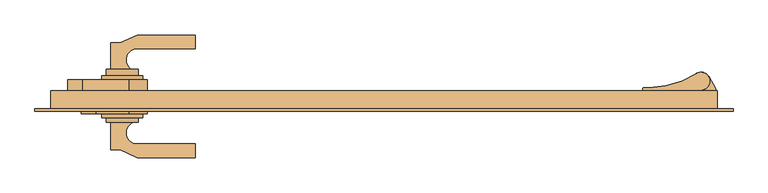
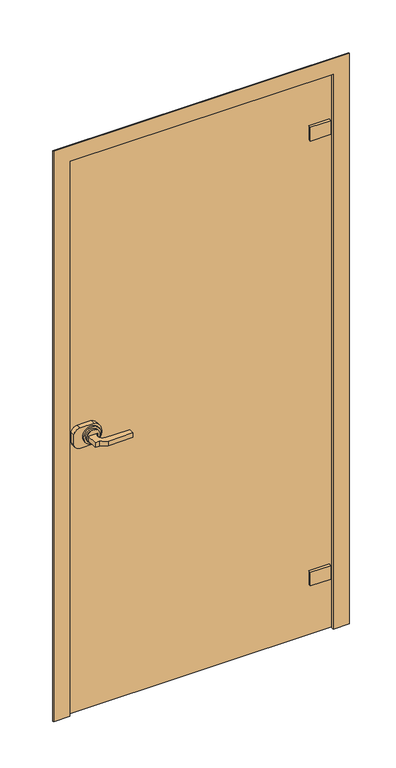
"""IFC4 building model written with IfcOpenShell, lengths in millimetres: door geometry, Doors_Doors_Faraone_Anta : Doors_Doors_Faraone_Anta."""

from ifc_helpers import new_model, si_unit, point, frame, frame_2d, origin, place, context, project, spatial, polyline, circle_curve, trimmed, segment, composite_curve, outline, extrude, faceted_brep, source, transform, mapped, element, save


def door_6f7413cf(model_context):
    return source(origin(), model_context, "Body", "SolidModel", [
        extrude(outline(polyline([(376.5509112, -11.599726), (376.5509112, -1.8997991), (446.250386, -1.8997991), (446.250386, -11.599726), (376.5509112, -11.599726)])), frame((0.0, 0.0, 1799.0000277), z_axis=(0.0, 0.0, 1.0), x_axis=(1.0, 0.0, 0.0)), (0.0, 0.0, 1.0), 50.0),
        extrude(outline(composite_curve([segment(trimmed(circle_curve(frame_2d((378.5508961, 17.600054)), 1.9999849), [point((376.5509112, 17.600054))], [point((378.5508961, 19.6000389))], False, "CARTESIAN"), True, "CONTINUOUS"), segment(polyline([(378.5508961, 19.6000389), (386.5508359, 19.6000389)]), True, "CONTINUOUS"), segment(trimmed(circle_curve(frame_2d((385.1363002, 147.5843675)), 127.9921454), [point((386.5508359, 19.6000389))], [point((454.7624862, 40.1870515))], True, "CARTESIAN"), True, "CONTINUOUS"), segment(trimmed(circle_curve(frame_2d((461.5502708, 29.0999673)), 12.9999021), [point((454.7624862, 40.1870515))], [point((466.1896331, 16.9560894))], False, "CARTESIAN"), True, "CONTINUOUS"), segment(polyline([(466.1896331, 16.9560894), (446.5503838, 9.6001143), (446.5503838, 8.1001256), (376.5509112, 8.1001256), (376.5509112, 17.600054)]), True, "CONTINUOUS")], self_intersect=False)), frame((0.0, 0.0, 1799.0000277), z_axis=(0.0, 0.0, 1.0), x_axis=(1.0, 0.0, 0.0)), (0.0, 0.0, 1.0), 50.0),
        extrude(outline(composite_curve([segment(polyline([(483.3501065, 18.0609582), (483.3501065, 15.0000736), (461.5537493, 15.0000736), (457.1671339, 16.861276)]), True, "CONTINUOUS"), segment(trimmed(circle_curve(frame_2d((461.5502708, 29.0999673)), 12.9999021), [point((457.1671339, 16.861276))], [point((451.2009633, 36.9669419))], False, "CARTESIAN"), True, "CONTINUOUS"), segment(trimmed(circle_curve(frame_2d((461.5502708, 29.0999673)), 12.9999021), [point((451.2009633, 36.9669419))], [point((472.573012, 35.9917471))], False, "CARTESIAN"), True, "CONTINUOUS"), segment(polyline([(472.573012, 35.9917471), (483.3501065, 18.0609582)]), True, "CONTINUOUS")], self_intersect=False)), frame((0.0, 0.0, 1749.0000277), z_axis=(0.0, 0.0, 1.0), x_axis=(1.0, 0.0, 0.0)), (0.0, 0.0, 1.0), 50.0),
        extrude(outline(polyline([(376.5509112, -11.599726), (376.5509112, -1.8997991), (446.250386, -1.8997991), (446.250386, -11.599726), (376.5509112, -11.599726)])), frame((0.0, 0.0, 182.0), z_axis=(0.0, 0.0, 1.0), x_axis=(1.0, 0.0, 0.0)), (0.0, 0.0, 1.0), 50.0),
        extrude(outline(composite_curve([segment(trimmed(circle_curve(frame_2d((378.5508961, 17.600054)), 1.9999849), [point((376.5509112, 17.600054))], [point((378.5508961, 19.6000389))], False, "CARTESIAN"), True, "CONTINUOUS"), segment(polyline([(378.5508961, 19.6000389), (386.5508359, 19.6000389)]), True, "CONTINUOUS"), segment(trimmed(circle_curve(frame_2d((385.1363002, 147.5843675)), 127.9921454), [point((386.5508359, 19.6000389))], [point((454.7624862, 40.1870515))], True, "CARTESIAN"), True, "CONTINUOUS"), segment(trimmed(circle_curve(frame_2d((461.5502708, 29.0999673)), 12.9999021), [point((454.7624862, 40.1870515))], [point((466.1896331, 16.9560894))], False, "CARTESIAN"), True, "CONTINUOUS"), segment(polyline([(466.1896331, 16.9560894), (446.5503838, 9.6001143), (446.5503838, 8.1001256), (376.5509112, 8.1001256), (376.5509112, 17.600054)]), True, "CONTINUOUS")], self_intersect=False)), frame((0.0, 0.0, 182.0), z_axis=(0.0, 0.0, 1.0), x_axis=(1.0, 0.0, 0.0)), (0.0, 0.0, 1.0), 50.0),
        extrude(outline(composite_curve([segment(polyline([(483.3501065, 18.0609582), (483.3501065, 15.0000736), (461.5537493, 15.0000736), (457.1671339, 16.861276)]), True, "CONTINUOUS"), segment(trimmed(circle_curve(frame_2d((461.5502708, 29.0999673)), 12.9999021), [point((457.1671339, 16.861276))], [point((451.2009633, 36.9669419))], False, "CARTESIAN"), True, "CONTINUOUS"), segment(trimmed(circle_curve(frame_2d((461.5502708, 29.0999673)), 12.9999021), [point((451.2009633, 36.9669419))], [point((472.573012, 35.9917471))], False, "CARTESIAN"), True, "CONTINUOUS"), segment(polyline([(472.573012, 35.9917471), (483.3501065, 18.0609582)]), True, "CONTINUOUS")], self_intersect=False)), frame((0.0, 0.0, 132.0), z_axis=(0.0, 0.0, 1.0), x_axis=(1.0, 0.0, 0.0)), (0.0, 0.0, 1.0), 50.0),
        extrude(outline(composite_curve([segment(trimmed(circle_curve(frame_2d((1003.2884985, -381.2459675)), 23.0897305), [point((1003.2884985, -404.335698))], [point((1003.2884985, -358.156237))], False, "CARTESIAN"), True, "CONTINUOUS"), segment(trimmed(circle_curve(frame_2d((1003.2884985, -381.2459675)), 23.0897305), [point((1003.2884985, -358.156237))], [point((1003.2884985, -404.335698))], False, "CARTESIAN"), True, "CONTINUOUS")], self_intersect=False)), frame((0.0, 36.9863146, 0.0), z_axis=(0.0, 1.0, 0.0), x_axis=(0.0, 0.0, 1.0)), (0.0, 0.0, 1.0), 9.3686894),
        extrude(outline(composite_curve([segment(trimmed(circle_curve(frame_2d((987.7717852, -438.83347)), 22.4105262), [point((983.5880679, -460.8500137))], [point((965.361259, -438.83347))], False, "CARTESIAN"), True, "CONTINUOUS"), segment(polyline([(965.361259, -438.83347), (965.361259, -373.83347)]), True, "CONTINUOUS"), segment(trimmed(circle_curve(frame_2d((1002.861259, -383.4990023)), 38.7256054), [point((965.361259, -373.83347))], [point((1039.5100566, -370.9874819))], False, "CARTESIAN"), True, "CONTINUOUS"), segment(polyline([(1039.5100566, -370.9874819), (1039.5100566, -438.83347)]), True, "CONTINUOUS"), segment(trimmed(circle_curve(frame_2d((1017.0995304, -438.83347)), 22.4105262), [point((1039.5100566, -438.83347))], [point((1021.2832478, -460.8500137))], False, "CARTESIAN"), True, "CONTINUOUS"), segment(polyline([(1021.2832478, -460.8500137), (983.5880679, -460.8500137)]), True, "CONTINUOUS")], self_intersect=False)), frame((0.0, 8.1001256, 0.0), z_axis=(0.0, 1.0, 0.0), x_axis=(0.0, 0.0, 1.0)), (0.0, 0.0, 1.0), 23.0652027),
        extrude(outline(composite_curve([segment(trimmed(circle_curve(frame_2d((987.7717852, -438.83347)), 22.4105262), [point((983.5880679, -460.8500137))], [point((965.361259, -438.83347))], False, "CARTESIAN"), True, "CONTINUOUS"), segment(polyline([(965.361259, -438.83347), (965.361259, -373.83347)]), True, "CONTINUOUS"), segment(trimmed(circle_curve(frame_2d((1002.861259, -383.4990023)), 38.7256054), [point((965.361259, -373.83347))], [point((1039.5100566, -370.9874819))], False, "CARTESIAN"), True, "CONTINUOUS"), segment(polyline([(1039.5100566, -370.9874819), (1039.5100566, -438.83347)]), True, "CONTINUOUS"), segment(trimmed(circle_curve(frame_2d((1017.0995304, -438.83347)), 22.4105262), [point((1039.5100566, -438.83347))], [point((1021.2832478, -460.8500137))], False, "CARTESIAN"), True, "CONTINUOUS"), segment(polyline([(1021.2832478, -460.8500137), (983.5880679, -460.8500137)]), True, "CONTINUOUS")], self_intersect=False)), frame((0.0, 8.1001256, 0.0), z_axis=(0.0, 1.0, 0.0), x_axis=(0.0, 0.0, 1.0)), (0.0, 0.0, 1.0), 23.0652027),
        extrude(outline(composite_curve([segment(trimmed(circle_curve(frame_2d((1003.2884985, -381.2459675)), 30.0), [point((1003.2884985, -411.2459675))], [point((1003.2884985, -351.2459675))], False, "CARTESIAN"), True, "CONTINUOUS"), segment(trimmed(circle_curve(frame_2d((1003.2884985, -381.2459675)), 30.0), [point((1003.2884985, -351.2459675))], [point((1003.2884985, -411.2459675))], False, "CARTESIAN"), True, "CONTINUOUS")], self_intersect=False)), frame((0.0, 31.1653283, 0.0), z_axis=(0.0, 1.0, 0.0), x_axis=(0.0, 0.0, 1.0)), (0.0, 0.0, 1.0), 5.8209863),
        extrude(outline(composite_curve([segment(trimmed(circle_curve(frame_2d((987.7717852, -438.83347)), 22.4105262), [point((983.5880679, -460.8500137))], [point((965.361259, -438.83347))], False, "CARTESIAN"), True, "CONTINUOUS"), segment(polyline([(965.361259, -438.83347), (965.361259, -373.83347)]), True, "CONTINUOUS"), segment(trimmed(circle_curve(frame_2d((1002.861259, -383.4990023)), 38.7256054), [point((965.361259, -373.83347))], [point((1039.5100566, -370.9874819))], False, "CARTESIAN"), True, "CONTINUOUS"), segment(polyline([(1039.5100566, -370.9874819), (1039.5100566, -438.83347)]), True, "CONTINUOUS"), segment(trimmed(circle_curve(frame_2d((1017.0995304, -438.83347)), 22.4105262), [point((1039.5100566, -438.83347))], [point((1021.2832478, -460.8500137))], False, "CARTESIAN"), True, "CONTINUOUS"), segment(polyline([(1021.2832478, -460.8500137), (983.5880679, -460.8500137)]), True, "CONTINUOUS")], self_intersect=False)), frame((0.0, 8.1001256, 0.0), z_axis=(0.0, 1.0, 0.0), x_axis=(0.0, 0.0, 1.0)), (0.0, 0.0, 1.0), 23.0652027),
        extrude(outline(composite_curve([segment(trimmed(circle_curve(frame_2d((1003.2884985, -381.2459675)), 23.0897305), [point((1003.2884985, -404.335698))], [point((1003.2884985, -358.156237))], False, "CARTESIAN"), True, "CONTINUOUS"), segment(trimmed(circle_curve(frame_2d((1003.2884985, -381.2459675)), 23.0897305), [point((1003.2884985, -358.156237))], [point((1003.2884985, -404.335698))], False, "CARTESIAN"), True, "CONTINUOUS")], self_intersect=False)), frame((0.0, 32.1653283, 0.0), z_axis=(0.0, 1.0, 0.0), x_axis=(0.0, 0.0, 1.0)), (0.0, 0.0, 1.0), 14.1896757),
        extrude(outline(composite_curve([segment(trimmed(circle_curve(frame_2d((987.7717852, -438.83347)), 22.4105262), [point((983.5880679, -460.8500137))], [point((965.361259, -438.83347))], False, "CARTESIAN"), True, "CONTINUOUS"), segment(polyline([(965.361259, -438.83347), (965.361259, -373.83347)]), True, "CONTINUOUS"), segment(trimmed(circle_curve(frame_2d((1002.861259, -383.4990023)), 38.7256054), [point((965.361259, -373.83347))], [point((1039.5100566, -370.9874819))], False, "CARTESIAN"), True, "CONTINUOUS"), segment(polyline([(1039.5100566, -370.9874819), (1039.5100566, -438.83347)]), True, "CONTINUOUS"), segment(trimmed(circle_curve(frame_2d((1017.0995304, -438.83347)), 22.4105262), [point((1039.5100566, -438.83347))], [point((1021.2832478, -460.8500137))], False, "CARTESIAN"), True, "CONTINUOUS"), segment(polyline([(1021.2832478, -460.8500137), (983.5880679, -460.8500137)]), True, "CONTINUOUS")], self_intersect=False)), frame((0.0, 8.1001256, 0.0), z_axis=(0.0, 1.0, 0.0), x_axis=(0.0, 0.0, 1.0)), (0.0, 0.0, 1.0), 23.0652027),
        extrude(outline(composite_curve([segment(trimmed(circle_curve(frame_2d((987.7717852, -438.83347)), 22.4105262), [point((983.5880679, -460.8500137))], [point((965.361259, -438.83347))], False, "CARTESIAN"), True, "CONTINUOUS"), segment(polyline([(965.361259, -438.83347), (965.361259, -373.83347)]), True, "CONTINUOUS"), segment(trimmed(circle_curve(frame_2d((1002.861259, -383.4990023)), 38.7256054), [point((965.361259, -373.83347))], [point((1039.5100566, -370.9874819))], False, "CARTESIAN"), True, "CONTINUOUS"), segment(polyline([(1039.5100566, -370.9874819), (1039.5100566, -438.83347)]), True, "CONTINUOUS"), segment(trimmed(circle_curve(frame_2d((1017.0995304, -438.83347)), 22.4105262), [point((1039.5100566, -438.83347))], [point((1021.2832478, -460.8500137))], False, "CARTESIAN"), True, "CONTINUOUS"), segment(polyline([(1021.2832478, -460.8500137), (983.5880679, -460.8500137)]), True, "CONTINUOUS")], self_intersect=False)), frame((0.0, 8.1001256, 0.0), z_axis=(0.0, 1.0, 0.0), x_axis=(0.0, 0.0, 1.0)), (0.0, 0.0, 1.0), 23.0652027),
        extrude(outline(composite_curve([segment(polyline([(-397.6805645, 84.9663543), (-383.9984574, 84.9663543), (-359.5544088, 96.3648014), (-274.5544088, 96.3648014), (-274.5544088, 76.3648014), (-359.5544088, 76.3648014)]), True, "CONTINUOUS"), segment(trimmed(circle_curve(frame_2d((-359.5544088, 60.2485058)), 16.1162956), [point((-359.5544088, 76.3648014))], [point((-367.7217579, 46.355004))], True, "CARTESIAN"), True, "CONTINUOUS"), segment(polyline([(-367.7217579, 46.355004), (-397.6805645, 46.355004), (-397.6805645, 84.9663543)]), True, "CONTINUOUS")], self_intersect=False)), frame((0.0, 0.0, 992.5658854), z_axis=(0.0, 0.0, 1.0), x_axis=(1.0, 0.0, 0.0)), (0.0, 0.0, 1.0), 16.6938628),
        extrude(outline(composite_curve([segment(trimmed(circle_curve(frame_2d((987.7717852, -438.83347)), 22.4105262), [point((983.5880679, -460.8500137))], [point((965.361259, -438.83347))], False, "CARTESIAN"), True, "CONTINUOUS"), segment(polyline([(965.361259, -438.83347), (965.361259, -373.83347)]), True, "CONTINUOUS"), segment(trimmed(circle_curve(frame_2d((1002.861259, -383.4990023)), 38.7256054), [point((965.361259, -373.83347))], [point((1039.5100566, -370.9874819))], False, "CARTESIAN"), True, "CONTINUOUS"), segment(polyline([(1039.5100566, -370.9874819), (1039.5100566, -438.83347)]), True, "CONTINUOUS"), segment(trimmed(circle_curve(frame_2d((1017.0995304, -438.83347)), 22.4105262), [point((1039.5100566, -438.83347))], [point((1021.2832478, -460.8500137))], False, "CARTESIAN"), True, "CONTINUOUS"), segment(polyline([(1021.2832478, -460.8500137), (983.5880679, -460.8500137)]), True, "CONTINUOUS")], self_intersect=False)), frame((0.0, 8.1001256, 0.0), z_axis=(0.0, 1.0, 0.0), x_axis=(0.0, 0.0, 1.0)), (0.0, 0.0, 1.0), 23.0652027),
        extrude(outline(composite_curve([segment(trimmed(circle_curve(frame_2d((1003.2884985, -381.2459675)), 23.0897305), [point((1003.2884985, -404.335698))], [point((1003.2884985, -358.156237))], False, "CARTESIAN"), True, "CONTINUOUS"), segment(trimmed(circle_curve(frame_2d((1003.2884985, -381.2459675)), 23.0897305), [point((1003.2884985, -358.156237))], [point((1003.2884985, -404.335698))], False, "CARTESIAN"), True, "CONTINUOUS")], self_intersect=False)), frame((0.0, -30.8998744, 0.0), z_axis=(0.0, 1.0, 0.0), x_axis=(0.0, 0.0, 1.0)), (0.0, 0.0, 1.0), 7.0),
        extrude(outline(composite_curve([segment(trimmed(circle_curve(frame_2d((987.7717852, -418.83347)), 22.4105262), [point((983.5880679, -440.8500137))], [point((965.361259, -418.83347))], False, "CARTESIAN"), True, "CONTINUOUS"), segment(polyline([(965.361259, -418.83347), (965.361259, -373.83347)]), True, "CONTINUOUS"), segment(trimmed(circle_curve(frame_2d((1002.861259, -383.4990023)), 38.7256054), [point((965.361259, -373.83347))], [point((1039.5100566, -370.9874819))], False, "CARTESIAN"), True, "CONTINUOUS"), segment(polyline([(1039.5100566, -370.9874819), (1039.5100566, -418.83347)]), True, "CONTINUOUS"), segment(trimmed(circle_curve(frame_2d((1017.0995304, -418.83347)), 22.4105262), [point((1039.5100566, -418.83347))], [point((1021.2832478, -440.8500137))], False, "CARTESIAN"), True, "CONTINUOUS"), segment(polyline([(1021.2832478, -440.8500137), (983.5880679, -440.8500137)]), True, "CONTINUOUS")], self_intersect=False)), frame((0.0, -17.8998744, 0.0), z_axis=(0.0, 1.0, 0.0), x_axis=(0.0, 0.0, 1.0)), (0.0, 0.0, 1.0), 16.0),
        extrude(outline(composite_curve([segment(polyline([(-397.6805645, -70.762087), (-397.6805645, -30.8998744), (-365.0665065, -30.8998744)]), True, "CONTINUOUS"), segment(trimmed(circle_curve(frame_2d((-359.5544088, -46.0442385)), 16.1162956), [point((-365.0665065, -30.8998744))], [point((-359.5544088, -62.1605341))], True, "CARTESIAN"), True, "CONTINUOUS"), segment(polyline([(-359.5544088, -62.1605341), (-274.5544088, -62.1605341), (-274.5544088, -82.1605341), (-359.5544088, -82.1605341), (-383.9984574, -70.762087), (-397.6805645, -70.762087)]), True, "CONTINUOUS")], self_intersect=False)), frame((0.0, 0.0, 992.5658854), z_axis=(0.0, 0.0, 1.0), x_axis=(1.0, 0.0, 0.0)), (0.0, 0.0, 1.0), 16.6938628),
        extrude(outline(composite_curve([segment(trimmed(circle_curve(frame_2d((1003.2884985, -381.2459675)), 30.0), [point((1003.2884985, -411.2459675))], [point((1003.2884985, -351.2459675))], False, "CARTESIAN"), True, "CONTINUOUS"), segment(trimmed(circle_curve(frame_2d((1003.2884985, -381.2459675)), 30.0), [point((1003.2884985, -351.2459675))], [point((1003.2884985, -411.2459675))], False, "CARTESIAN"), True, "CONTINUOUS")], self_intersect=False)), frame((0.0, -23.8998744, 0.0), z_axis=(0.0, 1.0, 0.0), x_axis=(0.0, 0.0, 1.0)), (0.0, 0.0, 1.0), 6.0),
        faceted_brep([(-452.3502762, -14.999774, 0.0), (-508.3498379, -14.999774, 0.0), (-508.3498379, -11.2997382, 0.0), (-499.0499489, -11.2997382, 0.0), (-499.0499489, -12.9997254, 0.0), (-485.3500137, -12.9997254, 0.0), (-485.3500137, 15.0, 0.0), (-467.3501757, 15.0, 0.0), (-467.3501757, -5.9998078, 0.0), (-452.3502762, -5.9998078, 0.0), (-452.3502762, -5.9998078, 2017.0002901), (-452.3502762, -14.999774, 2017.0002901), (-467.3501757, -5.9998078, 2032.0001896), (467.3501757, -5.9998078, 2032.0001896), (467.3501757, -5.9998078, 0.0), (452.3502762, -5.9998078, 0.0), (452.3502762, -5.9998078, 2017.0002901), (-467.3501757, 15.0, 2032.0001896), (-485.3500137, 15.0, 2050.0000277), (485.3500137, 15.0, 2050.0000277), (485.3500137, 15.0, 0.0), (467.3501757, 15.0, 0.0), (467.3501757, 15.0, 2032.0001896), (-485.3500137, -12.9997254, 2050.0000277), (-499.0499489, -12.9997254, 2063.6999629), (499.0499489, -12.9997254, 2063.6999629), (499.0499489, -12.9997254, 0.0), (485.3500137, -12.9997254, 0.0), (485.3500137, -12.9997254, 2050.0000277), (-499.0499489, -11.2997382, 2063.6999629), (-508.3498379, -11.2997382, 2072.9998518), (508.3498379, -11.2997382, 2072.9998518), (508.3498379, -11.2997382, 0.0), (499.0499489, -11.2997382, 0.0), (499.0499489, -11.2997382, 2063.6999629), (-508.3498379, -14.999774, 2072.9998518), (452.3502762, -14.999774, 2017.0002901), (452.3502762, -14.999774, 0.0), (508.3498379, -14.999774, 0.0), (508.3498379, -14.999774, 2072.9998518)], [[[0, 1, 2, 3, 4, 5, 6, 7, 8, 9]], [[9, 10, 11, 0]], [[8, 12, 13, 14, 15, 16, 10, 9]], [[7, 17, 12, 8]], [[6, 18, 19, 20, 21, 22, 17, 7]], [[5, 23, 18, 6]], [[4, 24, 25, 26, 27, 28, 23, 5]], [[3, 29, 24, 4]], [[2, 30, 31, 32, 33, 34, 29, 3]], [[1, 35, 30, 2]], [[0, 11, 36, 37, 38, 39, 35, 1]], [[16, 15, 37, 36]], [[37, 15, 14, 21, 20, 27, 26, 33, 32, 38]], [[22, 21, 14, 13]], [[28, 27, 20, 19]], [[34, 33, 26, 25]], [[39, 38, 32, 31]], [[10, 16, 36, 11]], [[17, 22, 13, 12]], [[23, 28, 19, 18]], [[29, 34, 25, 24]], [[35, 39, 31, 30]]]),
        extrude(outline(polyline([(0.0, -460.8500137), (0.0, 9.5), (0.0, 460.8500137), (2023.9998511, 460.8500137), (2023.9998511, -460.8500137), (0.0, -460.8500137)])), frame((0.0, -1.8998744, 0.0), z_axis=(0.0, 1.0, 0.0), x_axis=(0.0, 0.0, 1.0)), (0.0, 0.0, 1.0), 10.0),
    ])


if __name__ == "__main__":
    model = new_model("IFC4")
    model_context = context("Model", 3, world=origin())
    ifc_project = project(units=[si_unit("LENGTHUNIT", "METRE", prefix="MILLI")], contexts=[model_context])
    site = spatial("IfcSite", under=ifc_project)
    building = spatial("IfcBuilding", under=site)
    placement = place(None, origin())
    door_shape = door_6f7413cf(model_context)
    element("IfcDoor", 1, ObjectType="Doors_Doors_Faraone_Anta : Doors_Doors_Faraone_Anta", at=placement, inside=building, context=model_context, shape_type="MappedRepresentation", body=[
        mapped(door_shape, transform((0.0, 0.0, 0.0), x_axis=(1.0, 0.0, 0.0), y_axis=(0.0, 1.0, 0.0), z_axis=(0.0, 0.0, 1.0))),
    ])
    save(model, "model.ifc")

# Revit data of these elements
# Type "Doors_Doors_Faraone_Anta : Doors_Doors_Faraone_Anta"
#   Type Mark = "58"
#   URL = "https://faraone.it/en/"
#   Product data url = ""
#   Product Guid = ""
#   Model = "Spazio_Anta"
#   Manufacturer = "Faraone"
#   Keynote = "08110"
#   Assembly Code = "C1020100"
#   Analytic Construction = "<None>"
#   Width [instance default] = 1104.999 mm
#   Height [instance default] = 2700 mm
#   Handle Height = 1000 mm
#   Thickness = 11 mm
#   Glass Width [instance default] = 1055.999 mm
#   Middle Hinge [instance default] = yes
#   Edition number = 1
#   Define Thermal Properties by = 1
#   Interior Material = Glass - Faraone - Transparent
#   Handle Type = element 507032
#   Exterior Material = Aluminium - Faraone - Silver
#   Function = (empty or 0)
# Element 1 (IfcDoor, "Doors_Doors_Faraone_Anta : Doors_Doors_Faraone_Anta")
#   Width = 970.7 mm
#   Height = 2050 mm
#   Glass Width = 921.7 mm
#   Middle Hinge = no
#   Materials on its faces: "Aluminium - Faraone - Silver", "Glass - Faraone - Transparent"
# Materials
#   "Glass - Faraone - Transparent": class "Glass", colour RGB 0 128 192, transparency 0.9, Description = "Soda Lime Glass", Cost = 0
#   "Aluminium - Faraone - Silver": class "Metal", colour RGB 244 244 244, transparency 0, Description = "Metal - Faraone - Aluminium", Cost = 0
